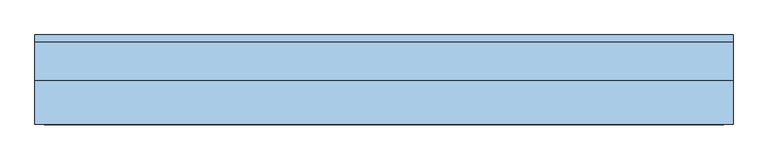
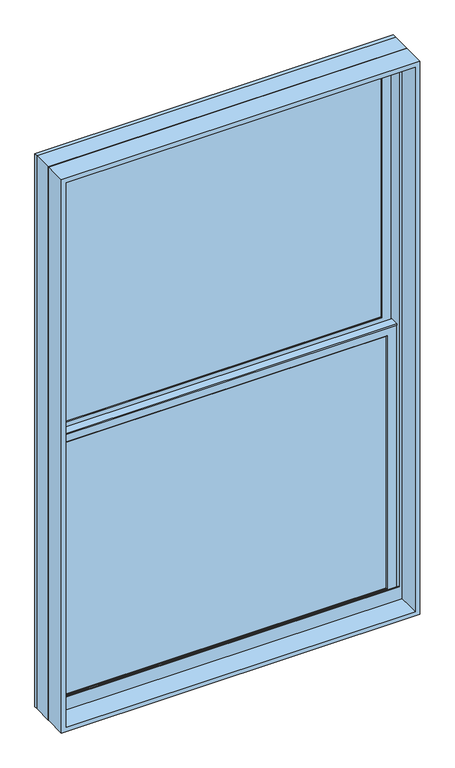
"""IFC4 building model written with IfcOpenShell, lengths in millimetres: window geometry, Window-Double_Hung-Marvin-Essential : ESDH4066."""

from ifc_helpers import new_model, si_unit, frame, origin, place, context, project, spatial, polyline, outline, extrude, faceted_brep, source, transform, mapped, element, save


def window_0ba9222f(model_context):
    return source(origin(), model_context, "Body", "SolidModel", [
        extrude(outline(polyline([(191.5583333, 20.6375), (191.5583333, 15.875), (172.5083333, 15.875), (172.5083333, 20.6375), (191.5583333, 20.6375)])), frame((0.0, 0.0, 527.05), z_axis=(0.0, 0.0, 1.0), x_axis=(1.0, 0.0, 0.0)), (0.0, 0.0, 1.0), 908.05),
        extrude(outline(polyline([(-172.5083333, 20.6375), (-172.5083333, 15.875), (-191.5583333, 15.875), (-191.5583333, 20.6375), (-172.5083333, 20.6375)])), frame((0.0, 0.0, 527.05), z_axis=(0.0, 0.0, 1.0), x_axis=(1.0, 0.0, 0.0)), (0.0, 0.0, 1.0), 908.05),
        extrude(outline(polyline([(546.1, 20.6375), (546.1, 15.875), (-546.1, 15.875), (-546.1, 20.6375), (546.1, 20.6375)])), frame((0.0, 0.0, 971.55), z_axis=(0.0, 0.0, 1.0), x_axis=(1.0, 0.0, 0.0)), (0.0, 0.0, 1.0), 19.05),
        extrude(outline(polyline([(-191.5583333, 46.83125), (-191.5583333, 51.59375), (-172.5083333, 51.59375), (-172.5083333, 46.83125), (-191.5583333, 46.83125)])), frame((0.0, 0.0, 1473.2), z_axis=(0.0, 0.0, 1.0), x_axis=(1.0, 0.0, 0.0)), (0.0, 0.0, 1.0), 908.05),
        extrude(outline(polyline([(172.5083333, 46.83125), (172.5083333, 51.59375), (191.5583333, 51.59375), (191.5583333, 46.83125), (172.5083333, 46.83125)])), frame((0.0, 0.0, 1473.2), z_axis=(0.0, 0.0, 1.0), x_axis=(1.0, 0.0, 0.0)), (0.0, 0.0, 1.0), 908.05),
        extrude(outline(polyline([(-546.1, 46.83125), (-546.1, 51.59375), (546.1, 51.59375), (546.1, 46.83125), (-546.1, 46.83125)])), frame((0.0, 0.0, 1917.7), z_axis=(0.0, 0.0, 1.0), x_axis=(1.0, 0.0, 0.0)), (0.0, 0.0, 1.0), 19.05),
        extrude(outline(polyline([(191.5583333, 20.6375), (172.5083333, 20.6375), (172.5083333, 25.4), (191.5583333, 25.4), (191.5583333, 20.6375)])), frame((0.0, 0.0, 527.05), z_axis=(0.0, 0.0, 1.0), x_axis=(1.0, 0.0, 0.0)), (0.0, 0.0, 1.0), 908.05),
        extrude(outline(polyline([(-172.5083333, 20.6375), (-191.5583333, 20.6375), (-191.5583333, 25.4), (-172.5083333, 25.4), (-172.5083333, 20.6375)])), frame((0.0, 0.0, 527.05), z_axis=(0.0, 0.0, 1.0), x_axis=(1.0, 0.0, 0.0)), (0.0, 0.0, 1.0), 908.05),
        extrude(outline(polyline([(546.1, 20.6375), (-546.1, 20.6375), (-546.1, 25.4), (546.1, 25.4), (546.1, 20.6375)])), frame((0.0, 0.0, 971.55), z_axis=(0.0, 0.0, 1.0), x_axis=(1.0, 0.0, 0.0)), (0.0, 0.0, 1.0), 19.05),
        extrude(outline(polyline([(-191.5583333, 56.35625), (-172.5083333, 56.35625), (-172.5083333, 51.59375), (-191.5583333, 51.59375), (-191.5583333, 56.35625)])), frame((0.0, 0.0, 1473.2), z_axis=(0.0, 0.0, 1.0), x_axis=(1.0, 0.0, 0.0)), (0.0, 0.0, 1.0), 908.05),
        extrude(outline(polyline([(172.5083333, 56.35625), (191.5583333, 56.35625), (191.5583333, 51.59375), (172.5083333, 51.59375), (172.5083333, 56.35625)])), frame((0.0, 0.0, 1473.2), z_axis=(0.0, 0.0, 1.0), x_axis=(1.0, 0.0, 0.0)), (0.0, 0.0, 1.0), 908.05),
        extrude(outline(polyline([(-546.1, 56.35625), (546.1, 56.35625), (546.1, 51.59375), (-546.1, 51.59375), (-546.1, 56.35625)])), frame((0.0, 0.0, 1917.7), z_axis=(0.0, 0.0, 1.0), x_axis=(1.0, 0.0, 0.0)), (0.0, 0.0, 1.0), 19.05),
        faceted_brep([(-573.0875, 5.6780605, 1465.1351748), (-573.0875, 5.6780605, 1460.5), (573.0875, 5.6780605, 1460.5), (573.0875, 5.6780605, 1465.1351748), (-573.0875, 34.8118605, 1465.1351748), (573.0875, 34.8118605, 1465.1351748), (573.0875, 34.8118605, 1460.5), (-573.0875, 34.8118605, 1460.5), (-573.0875, 30.1625, 1460.5), (-573.0875, 30.1625, 500.0625), (-573.0875, 8.9241104, 500.0625), (-573.0875, 8.9241104, 1460.5), (573.0875, 8.9241104, 1460.5), (573.0875, 30.1625, 1460.5), (573.0875, 8.9241104, 500.0625), (573.0875, 30.1625, 500.0625), (-557.2034752, 11.90625, 1446.2034752), (-557.2034752, 30.1625, 1446.2034752), (557.2034752, 30.1625, 1446.2034752), (557.2034752, 11.90625, 1446.2034752), (-540.54375, 10.4662439, 1429.54375), (-540.54375, 11.90625, 1429.54375), (540.54375, 11.90625, 1429.54375), (540.54375, 10.4662439, 1429.54375), (542.0858834, 8.9241104, 1431.0858834), (-542.0858834, 8.9241104, 1431.0858834), (557.2034752, 30.1625, 515.9465248), (557.2034752, 11.90625, 515.9465248), (540.54375, 11.90625, 532.60625), (540.54375, 10.4662439, 532.60625), (542.0858834, 8.9241104, 531.0641166), (-557.2034752, 30.1625, 515.9465248), (-557.2034752, 11.90625, 515.9465248), (-540.54375, 11.90625, 532.60625), (-540.54375, 10.4662439, 532.60625), (-542.0858834, 8.9241104, 531.0641166)], [[[0, 1, 2, 3]], [[4, 5, 6, 7]], [[1, 0, 4, 7, 8, 9, 10, 11]], [[2, 1, 11, 12]], [[7, 6, 13, 8]], [[3, 2, 12, 14, 15, 13, 6, 5]], [[0, 3, 5, 4]], [[16, 17, 18, 19]], [[20, 21, 22, 23]], [[20, 23, 24, 25]], [[19, 18, 26, 27]], [[23, 22, 28, 29]], [[24, 23, 29, 30]], [[27, 26, 31, 32]], [[29, 28, 33, 34]], [[30, 29, 34, 35]], [[15, 14, 10, 9]], [[15, 9, 8, 13], [18, 17, 31, 26]], [[17, 16, 32, 31]], [[16, 19, 27, 32], [22, 21, 33, 28]], [[21, 20, 34, 33]], [[20, 25, 35, 34]], [[10, 14, 12, 11], [25, 24, 30, 35]]]),
        extrude(outline(polyline([(38.5955581, 1446.2125), (33.5778968, 1446.2125), (33.5778968, 1447.8), (39.9405976, 1447.8), (39.9405976, 1446.2125), (61.515625, 1446.2125), (47.6307501, 1442.8975159), (38.5955581, 1442.8975159), (38.5955581, 1446.2125)])), frame((-573.0875, 0.0, 0.0), z_axis=(1.0, 0.0, 0.0), x_axis=(0.0, 1.0, 0.0)), (0.0, 0.0, 1.0), 1146.175),
        faceted_brep([(603.25, 0.0, 469.9), (603.25, 0.0, 2438.4), (-603.25, 0.0, 2438.4), (-603.25, 0.0, 469.9), (577.05625, 0.0, 531.01875), (-577.05625, 0.0, 531.01875), (-577.05625, 0.0, 2412.20625), (577.05625, 0.0, 2412.20625), (577.05625, 3.96875, 469.9), (-577.05625, 3.96875, 469.9), (-577.05625, 3.96875, 531.01875), (577.05625, 3.96875, 531.01875), (-603.25, 65.6828125, 469.9), (-577.05625, 65.6828125, 469.9), (577.05625, 65.6828125, 469.9), (603.25, 65.6828125, 469.9), (-603.25, 65.6828125, 2438.4), (603.25, 65.6828125, 2438.4), (577.05625, 65.6828125, 2412.20625), (-577.05625, 65.6828125, 2412.20625)], [[[0, 1, 2, 3], [4, 5, 6, 7]], [[8, 9, 10, 11]], [[5, 4, 11, 10]], [[0, 3, 12, 13, 9, 8, 14, 15]], [[13, 12, 16, 17, 15, 14, 18, 19]], [[13, 19, 6, 5, 10, 9]], [[7, 6, 19, 18]], [[18, 14, 8, 11, 4, 7]], [[1, 0, 15, 17]], [[2, 1, 17, 16]], [[3, 2, 16, 12]]]),
        faceted_brep([(577.05625, 30.1625, 1454.15), (575.46875, 30.1625, 1454.15), (575.46875, 30.1625, 494.2544613), (577.05625, 30.1625, 494.2544613), (-575.46875, 30.1625, 1454.15), (-577.05625, 30.1625, 1454.15), (-577.05625, 30.1625, 494.2544613), (-575.46875, 30.1625, 494.2544613), (575.46875, 63.5, 1454.15), (577.05625, 63.5, 1454.15), (577.05625, 63.5, 487.7743077), (575.46875, 63.5, 487.7743077), (-577.05625, 63.5, 1454.15), (-575.46875, 63.5, 1454.15), (-575.46875, 63.5, 487.7743077), (-577.05625, 63.5, 487.7743077), (588.3108932, 3.96875, 499.3460105), (588.3108932, 3.96875, 469.9), (588.3108932, 65.6828125, 469.9), (588.3108932, 65.6828125, 487.350012), (-588.3108932, 3.96875, 469.9), (-588.3108932, 3.96875, 499.3460105), (-588.3108932, 65.6828125, 487.350012), (-588.3108932, 65.6828125, 469.9), (588.3108932, 78.58125, 484.8428097), (-588.3108932, 78.58125, 484.8428097), (-586.2971252, 68.2348864, 486.8539391), (-568.33135, 68.2348864, 486.8539391), (-568.33135, 65.6828125, 487.350012), (568.33135, 65.6828125, 487.350012), (568.33135, 68.2348864, 486.8539391), (586.2971252, 68.2348864, 486.8539391), (-603.25, 65.6828125, 469.9), (-603.25, 78.5948249, 469.9), (603.25, 78.5948249, 469.9), (603.25, 65.6828125, 469.9), (-603.25, 78.58125, 2438.4), (603.25, 78.58125, 2438.4), (588.3108932, 78.58125, 2423.4608932), (-588.3108932, 78.58125, 2423.4608932), (-603.25, 65.6828125, 2438.4), (-586.2971252, 68.2348864, 2421.4471252), (586.2971252, 68.2348864, 2421.4471252), (568.33135, 68.2348864, 2403.48135), (-568.33135, 68.2348864, 2403.48135), (-568.33135, 65.6828125, 2403.48135), (568.33135, 65.6828125, 2403.48135), (603.25, 65.6828125, 2438.4)], [[[0, 1, 2, 3]], [[4, 5, 6, 7]], [[8, 9, 10, 11]], [[12, 13, 14, 15]], [[1, 8, 11, 2]], [[9, 0, 3, 10]], [[1, 0, 9, 8]], [[5, 4, 13, 12]], [[5, 12, 15, 6]], [[13, 4, 7, 14]], [[16, 17, 18, 19]], [[20, 21, 22, 23]], [[24, 25, 26, 27, 28, 22, 21, 16, 19, 29, 30, 31], [3, 2, 11, 10], [7, 6, 15, 14]], [[17, 16, 21, 20]], [[17, 20, 23, 32, 33, 34, 35, 18]], [[34, 33, 36, 37], [25, 24, 38, 39]], [[33, 32, 40, 36]], [[39, 41, 26, 25]], [[41, 42, 31, 30, 43, 44, 27, 26]], [[44, 45, 28, 27]], [[40, 32, 23, 22, 28, 45, 46, 29, 19, 18, 35, 47]], [[36, 40, 47, 37]], [[39, 38, 42, 41]], [[44, 43, 46, 45]], [[34, 37, 47, 35]], [[42, 38, 24, 31]], [[46, 43, 30, 29]]]),
        extrude(outline(polyline([(553.24375, 11.90625), (-553.24375, 11.90625), (-553.24375, 15.08125), (553.24375, 15.08125), (553.24375, 11.90625)])), frame((0.0, 0.0, 519.90625), z_axis=(0.0, 0.0, 1.0), x_axis=(1.0, 0.0, 0.0)), (0.0, 0.0, 1.0), 922.3375),
        extrude(outline(polyline([(553.24375, 42.8625), (-553.24375, 42.8625), (-553.24375, 46.0375), (553.24375, 46.0375), (553.24375, 42.8625)])), frame((0.0, 0.0, 1466.05625), z_axis=(0.0, 0.0, 1.0), x_axis=(1.0, 0.0, 0.0)), (0.0, 0.0, 1.0), 922.3375),
        faceted_brep([(-540.54375, 31.194477, 1429.54375), (-542.0858834, 32.7366104, 1431.0858834), (542.0858834, 32.7366104, 1431.0858834), (540.54375, 31.194477, 1429.54375), (-540.54375, 30.1625, 1429.54375), (540.54375, 30.1625, 1429.54375), (-573.0875, 32.7366104, 1462.0875), (-573.0875, 30.1625, 1462.0875), (573.0875, 30.1625, 1462.0875), (573.0875, 32.7366104, 1462.0875), (542.0858834, 32.7366104, 531.0641166), (540.54375, 31.194477, 532.60625), (540.54375, 30.1625, 532.60625), (573.0875, 30.1625, 500.0625), (573.0875, 32.7366104, 500.0625), (-542.0858834, 32.7366104, 531.0641166), (-540.54375, 31.194477, 532.60625), (-540.54375, 30.1625, 532.60625), (-573.0875, 30.1625, 500.0625), (-573.0875, 32.7366104, 500.0625)], [[[0, 1, 2, 3]], [[4, 0, 3, 5]], [[6, 7, 8, 9]], [[3, 2, 10, 11]], [[5, 3, 11, 12]], [[9, 8, 13, 14]], [[11, 10, 15, 16]], [[12, 11, 16, 17]], [[14, 13, 18, 19]], [[9, 14, 19, 6], [1, 15, 10, 2]], [[16, 15, 1, 0]], [[17, 16, 0, 4]], [[7, 18, 13, 8], [5, 12, 17, 4]], [[19, 18, 7, 6]]]),
        faceted_brep([(-557.2034752, 42.8625, 2392.3534752), (-557.2034752, 61.11875, 2392.3534752), (557.2034752, 61.11875, 2392.3534752), (557.2034752, 42.8625, 2392.3534752), (-540.54375, 41.4224939, 2375.69375), (-540.54375, 42.8625, 2375.69375), (540.54375, 42.8625, 2375.69375), (540.54375, 41.4224939, 2375.69375), (-542.0858834, 39.8803604, 2377.2358834), (542.0858834, 39.8803604, 2377.2358834), (-573.0875, 61.11875, 2408.2375), (-573.0875, 39.8803604, 2408.2375), (573.0875, 39.8803604, 2408.2375), (573.0875, 61.11875, 2408.2375), (557.2034752, 61.11875, 1462.0965248), (557.2034752, 42.8625, 1462.0965248), (540.54375, 42.8625, 1478.75625), (540.54375, 41.4224939, 1478.75625), (542.0858834, 39.8803604, 1477.2141166), (573.0875, 39.8803604, 1446.2125), (573.0875, 61.11875, 1446.2125), (-557.2034752, 61.11875, 1462.0965248), (-557.2034752, 42.8625, 1462.0965248), (-540.54375, 42.8625, 1478.75625), (-540.54375, 41.4224939, 1478.75625), (-542.0858834, 39.8803604, 1477.2141166), (-573.0875, 39.8803604, 1446.2125), (-573.0875, 61.11875, 1446.2125)], [[[0, 1, 2, 3]], [[4, 5, 6, 7]], [[8, 4, 7, 9]], [[10, 11, 12, 13]], [[3, 2, 14, 15]], [[7, 6, 16, 17]], [[9, 7, 17, 18]], [[13, 12, 19, 20]], [[15, 14, 21, 22]], [[17, 16, 23, 24]], [[18, 17, 24, 25]], [[20, 19, 26, 27]], [[13, 20, 27, 10], [1, 21, 14, 2]], [[22, 21, 1, 0]], [[3, 15, 22, 0], [5, 23, 16, 6]], [[24, 23, 5, 4]], [[25, 24, 4, 8]], [[11, 26, 19, 12], [9, 18, 25, 8]], [[27, 26, 11, 10]]]),
        faceted_brep([(-573.0875, 61.11875, 1446.2125), (-573.0875, 63.6928604, 1446.2125), (573.0875, 63.6928604, 1446.2125), (573.0875, 61.11875, 1446.2125), (-540.54375, 62.150727, 1478.75625), (-540.54375, 61.11875, 1478.75625), (540.54375, 61.11875, 1478.75625), (540.54375, 62.150727, 1478.75625), (-542.0858834, 63.6928604, 1477.2141166), (542.0858834, 63.6928604, 1477.2141166), (573.0875, 63.6928604, 2408.2375), (573.0875, 61.11875, 2408.2375), (540.54375, 61.11875, 2375.69375), (540.54375, 62.150727, 2375.69375), (542.0858834, 63.6928604, 2377.2358834), (-573.0875, 63.6928604, 2408.2375), (-573.0875, 61.11875, 2408.2375), (-540.54375, 61.11875, 2375.69375), (-540.54375, 62.150727, 2375.69375), (-542.0858834, 63.6928604, 2377.2358834)], [[[0, 1, 2, 3]], [[4, 5, 6, 7]], [[8, 4, 7, 9]], [[3, 2, 10, 11]], [[7, 6, 12, 13]], [[9, 7, 13, 14]], [[11, 10, 15, 16]], [[13, 12, 17, 18]], [[14, 13, 18, 19]], [[16, 15, 1, 0]], [[3, 11, 16, 0], [5, 17, 12, 6]], [[18, 17, 5, 4]], [[19, 18, 4, 8]], [[1, 15, 10, 2], [9, 14, 19, 8]]]),
        extrude(outline(polyline([(553.24375, 26.19375), (-553.24375, 26.19375), (-553.24375, 30.1625), (553.24375, 30.1625), (553.24375, 26.19375)])), frame((0.0, 0.0, 519.90625), z_axis=(0.0, 0.0, 1.0), x_axis=(1.0, 0.0, 0.0)), (0.0, 0.0, 1.0), 922.3375),
        extrude(outline(polyline([(553.24375, 57.15), (-553.24375, 57.15), (-553.24375, 61.11875), (553.24375, 61.11875), (553.24375, 57.15)])), frame((0.0, 0.0, 1466.05625), z_axis=(0.0, 0.0, 1.0), x_axis=(1.0, 0.0, 0.0)), (0.0, 0.0, 1.0), 922.3375),
        extrude(outline(polyline([(2438.4, 603.25), (2438.4, -603.25), (469.9, -603.25), (469.9, 603.25), (2438.4, 603.25)]), holes=[polyline([(2422.525, 587.375), (485.775, 587.375), (485.775, -587.375), (2422.525, -587.375), (2422.525, 587.375)])]), frame((0.0, -76.2, 0.0), z_axis=(0.0, 1.0, 0.0), x_axis=(0.0, 0.0, 1.0)), (0.0, 0.0, 1.0), 75.40625),
    ])


if __name__ == "__main__":
    model = new_model("IFC4")
    model_context = context("Model", 3, world=origin())
    ifc_project = project(units=[si_unit("LENGTHUNIT", "METRE", prefix="MILLI")], contexts=[model_context])
    site = spatial("IfcSite", under=ifc_project)
    building = spatial("IfcBuilding", under=site)
    placement = place(None, origin())
    window_shape = window_0ba9222f(model_context)
    element("IfcWindow", 1, ObjectType="Window-Double_Hung-Marvin-Essential : ESDH4066", at=placement, inside=building, context=model_context, shape_type="MappedRepresentation", body=[
        mapped(window_shape, transform((0.0, 0.0, 0.0), x_axis=(1.0, 0.0, 0.0), y_axis=(0.0, 1.0, 0.0), z_axis=(0.0, 0.0, 1.0))),
    ])
    save(model, "model.ifc")

# Revit data of these elements
# Type "Window-Double_Hung-Marvin-Essential : ESDH4066"
#   Type Mark = "88"
#   Window Type = "Essential Double Hung"
#   Product data url = "https://bimobject.com/marvin-windows-and-doors/product/marvin-dhwau"
#   Product Guid = "c4a96547-874c-4385-91dc-a058adc19d98"
#   Frame = "All Ultrex"
#   Egress Window = "Yes"
#   URL = "www.marvin.com"
#   Model = "ESDH4066"
#   Manufacturer = "Marvin Windows and Doors"
#   Label Egress = "EGRESS WDW"
#   Glass Type = "IG Low E II with Argon"
#   Design Pressure = "DP30"
#   Description = "4878 DBHG"
#   Analytic Construction = "<None>"
#   Prairie Corner Width = 0' - 4"
#   Prairie Corner Height = 0' - 4"
#   Egress Width = 3' - 8 9/16"
#   Egress Height = 2' - 10 27/128"
#   Rough Width = 4' - 0"
#   Rough Height = 6' - 6"
#   Nominal Width = 4' - 0"
#   Nominal Height = 6' - 6"
#   Inset to Installation Flange [instance default] = 0' - 1"
#   Height = 6' - 5 1/2"
#   Egress Area = 10.587 SF
#   Default Head Height = 8' - 0"
#   Width = 3' - 11 1/2"
#   Daylight Area = 20.8748 SF
#   DLO Width = 3' - 6 9/16"
#   DLO Height = 2' - 11 5/16"
#   Muntins Top Sash = yes
#   Lites Wide Top Sash = 3
#   Lites Wide Bottom Sash = 3
#   Lites High Top Sash = 2
#   Lites High Bottom Sash = 2
#   Lite Cut Prairie 9 = no
#   Lite Cut HV Grid = yes
#   Muntins Bottom Sash = yes
#   Label Visibility = no
#   Jamb Extension Visibility = yes
#   Edition number = 1
#   Interior Material = Ultrex-Marvin-Stonewhite
#   Glazing Material = Glass-Marvin-IG Low E II with Argon
#   Cladding Material = Ultrex-Marvin-Pebblegray
#   Wall Closure = (empty or 0)
#   Assembly Code = ""
# Element 1 (IfcWindow, "Window-Double_Hung-Marvin-Essential : ESDH4066")
#   Materials on its faces: "Ultrex-Marvin-Pebblegray", "Ultrex-Marvin-Stonewhite", "Glass-Marvin-IG Low E II with Argon"
# Materials
#   "Ultrex-Marvin-Stonewhite": class "Paint", colour RGB 250 251 245, transparency 0
#   "Glass-Marvin-IG Low E II with Argon": class "Glass", colour RGB 0 128 192, transparency 0.85
#   "Ultrex-Marvin-Pebblegray": class "Paint", colour RGB 189 185 173, transparency 0
